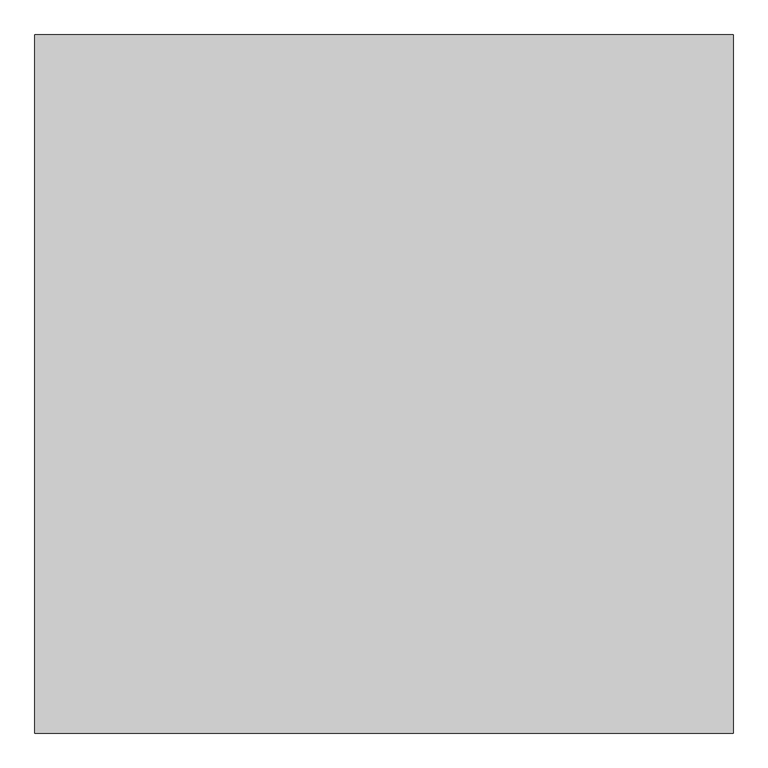
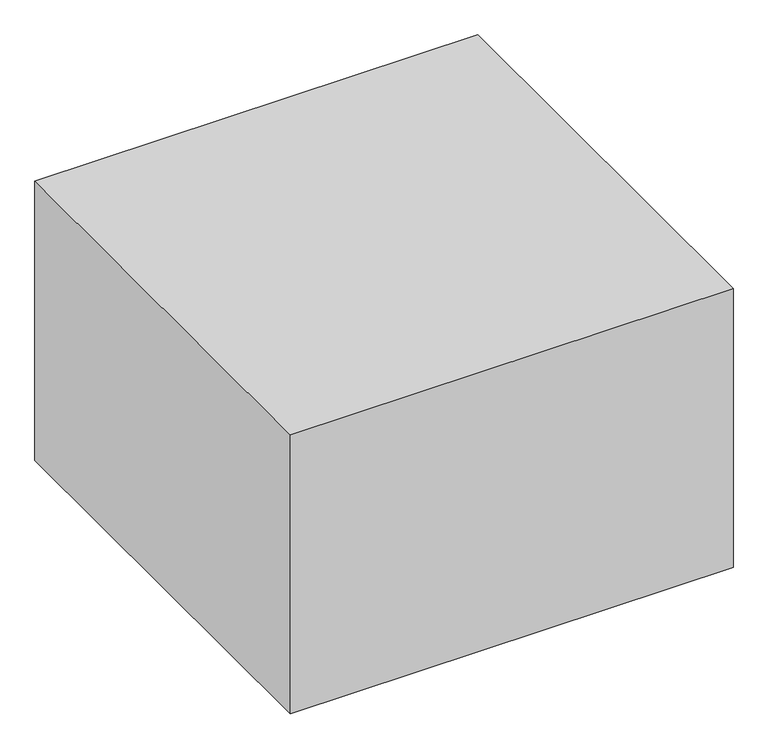
"""IFC4 building model written with IfcOpenShell, lengths in millimetres: proxy geometry, Space Planning Box_hec : Space Planning Box_hec."""

import ifcopenshell
import ifcopenshell.guid

model = None  # the IFC model being written
_history = None  # IfcOwnerHistory: only IFC2X3 demands one
_inside = {}  # id of a spatial element -> (the spatial element, [elements in it])
_under = {}  # id of a project, library or spatial element -> (it, [spatial elements below it])
_declared = {}  # id of a project -> (the project, [libraries it declares])
_typed = {}  # id of a type object -> (the type object, [elements of that type])
_made_of = {}  # id of a material, layer set ... -> (it, [elements and type objects made of it])


def new_model(schema):
    """Start an empty IFC model of exactly this schema.

    Asked for "IFC4X3", IfcOpenShell would pick the latest addendum, in which some entities
    have other attributes; the version numbers below select the first issue.
    IFC2X3 requires an IfcOwnerHistory on every rooted entity: one is made here for all.
    """
    global model, _history
    if schema == "IFC4X3":
        model = ifcopenshell.file(schema_version=(4, 3, 0, 0))
    else:
        model = ifcopenshell.file(schema=schema)
    _inside.clear()
    _under.clear()
    _declared.clear()
    _typed.clear()
    _made_of.clear()
    _history = None
    if model.schema == "IFC2X3":
        org = make("IfcOrganization", Name="unknown")
        user = make(
            "IfcPersonAndOrganization",
            ThePerson=make("IfcPerson", FamilyName="unknown"),
            TheOrganization=org,
        )
        app = make(
            "IfcApplication",
            ApplicationDeveloper=org,
            Version="unknown",
            ApplicationFullName="unknown",
            ApplicationIdentifier="unknown",
        )
        _history = make(
            "IfcOwnerHistory",
            OwningUser=user,
            OwningApplication=app,
            ChangeAction="ADDED",
            CreationDate=0,
        )
    return model


def make(cls, **values):
    """One entity of the class cls with the attributes given. An attribute that is None is left unset."""
    return model.create_entity(
        cls, **{name: value for name, value in values.items() if value is not None}
    )


def rooted(cls, **values):
    """An entity with a GlobalId (a new one), such as an element, a storey or a relation."""
    return make(cls, GlobalId=ifcopenshell.guid.new(), OwnerHistory=_history, **values)


def si_unit(unit_type, name, prefix=None):
    """IfcSIUnit, for example si_unit("LENGTHUNIT", "METRE", prefix="MILLI")."""
    return make("IfcSIUnit", UnitType=unit_type, Prefix=prefix, Name=name)


def assignment(units):
    """IfcUnitAssignment: the units of a project."""
    return None if units is None else make("IfcUnitAssignment", Units=units)


def point(xyz):
    """IfcCartesianPoint."""
    return None if xyz is None else make("IfcCartesianPoint", Coordinates=xyz)


def direction(xyz):
    """IfcDirection."""
    return None if xyz is None else make("IfcDirection", DirectionRatios=xyz)


def frame(location, z_axis=None, x_axis=None):
    """IfcAxis2Placement3D, a coordinate frame: its origin and axes. An axis left out is left unset."""
    return make(
        "IfcAxis2Placement3D",
        Location=point(location),
        Axis=direction(z_axis),
        RefDirection=direction(x_axis),
    )


def origin():
    """The frame at (0, 0, 0) with its axes left unset."""
    return frame((0.0, 0.0, 0.0))


def origin_with_axes():
    """The frame at (0, 0, 0) with the z axis (0, 0, 1) and the x axis (1, 0, 0) written out."""
    return frame((0.0, 0.0, 0.0), z_axis=(0.0, 0.0, 1.0), x_axis=(1.0, 0.0, 0.0))


def place(relative_to, where):
    """IfcLocalPlacement: puts the frame where relative to a parent placement (None: the world)."""
    return make(
        "IfcLocalPlacement", PlacementRelTo=relative_to, RelativePlacement=where
    )


def context(
    kind, dimensions, precision=None, world=None, true_north=None, identifier=None
):
    """IfcGeometricRepresentationContext, for example the 3D "Model" context."""
    return make(
        "IfcGeometricRepresentationContext",
        ContextIdentifier=identifier,
        ContextType=kind,
        CoordinateSpaceDimension=dimensions,
        Precision=precision,
        WorldCoordinateSystem=world,
        TrueNorth=true_north,
    )


def project(units=None, contexts=None):
    """IfcProject with its units and contexts."""
    return rooted(
        "IfcProject",
        Name="project",
        RepresentationContexts=contexts,
        UnitsInContext=assignment(units),
    )


def spatial(cls, under=None, at=None, **own):
    """A site, building, storey or space (cls), placed at a placement, below another one or the project."""
    s = rooted(cls, ObjectPlacement=at, **own)
    if under is not None:
        _under.setdefault(under.id(), (under, []))[1].append(s)
    return s


def polyline(points):
    """IfcPolyline through the points."""
    return make("IfcPolyline", Points=[point(p) for p in points])


def outline(outer, holes=None, kind="AREA"):
    """IfcArbitraryClosedProfileDef: a profile drawn as a closed curve; with holes, ...WithVoids."""
    if holes is None:
        return make("IfcArbitraryClosedProfileDef", ProfileType=kind, OuterCurve=outer)
    return make(
        "IfcArbitraryProfileDefWithVoids",
        ProfileType=kind,
        OuterCurve=outer,
        InnerCurves=holes,
    )


def extrude(swept, where, along, depth):
    """IfcExtrudedAreaSolid: the profile swept, set in the frame where, extruded along a direction by depth."""
    return make(
        "IfcExtrudedAreaSolid",
        SweptArea=swept,
        Position=where,
        ExtrudedDirection=direction(along),
        Depth=depth,
    )


def shape(context_of_items, identifier, shape_type, items):
    """IfcShapeRepresentation: the items that make up one representation, for example the "Body"."""
    return make(
        "IfcShapeRepresentation",
        ContextOfItems=context_of_items,
        RepresentationIdentifier=identifier,
        RepresentationType=shape_type,
        Items=items,
    )


def source(mapping_origin, context_of_items, identifier, shape_type, items):
    """IfcRepresentationMap: a shape defined once, which mapped items show again and again."""
    return make(
        "IfcRepresentationMap",
        MappingOrigin=mapping_origin,
        MappedRepresentation=shape(context_of_items, identifier, shape_type, items),
    )


def transform(
    local_origin,
    x_axis=None,
    y_axis=None,
    z_axis=None,
    scale=None,
    scale2=None,
    scale3=None,
    uniform=True,
):
    """IfcCartesianTransformationOperator3D, or its non-uniform kind. x_axis, y_axis, z_axis: its Axis1, 2, 3."""
    if uniform:
        return make(
            "IfcCartesianTransformationOperator3D",
            Axis1=direction(x_axis),
            Axis2=direction(y_axis),
            LocalOrigin=point(local_origin),
            Scale=scale,
            Axis3=direction(z_axis),
        )
    return make(
        "IfcCartesianTransformationOperator3DnonUniform",
        Axis1=direction(x_axis),
        Axis2=direction(y_axis),
        LocalOrigin=point(local_origin),
        Scale=scale,
        Axis3=direction(z_axis),
        Scale2=scale2,
        Scale3=scale3,
    )


def mapped(mapping_source, mapping_target):
    """IfcMappedItem: shows the shape of a source again, moved by a transform."""
    return make(
        "IfcMappedItem", MappingSource=mapping_source, MappingTarget=mapping_target
    )


def made_of(thing, what):
    """Note that an element or type object is made of a material, layer set ...; save() writes the relation."""
    if what is not None:
        _made_of.setdefault(what.id(), (what, []))[1].append(thing)
    return thing


def element(
    cls,
    number,
    at=None,
    inside=None,
    cuts=None,
    type_object=None,
    material=None,
    context=None,
    identifier="Body",
    shape_type=None,
    held_by="IfcProductDefinitionShape",
    body=None,
    shapes=None,
    **own,
):
    """One element of the class cls, such as IfcWall. Its Tag is "e" and its number.

    at: its placement. inside: the storey or other place that contains it. cuts: it is an
    opening in that element (IfcRelVoidsElement). A single representation is given by context,
    identifier, shape_type and body (its items); several are given by shapes. held_by: the class
    of the entity that holds the representations. save() writes the other relations.
    """
    e = rooted(cls, Tag="e%d" % number, ObjectPlacement=at, **own)
    if body is not None:
        shapes = [shape(context, identifier, shape_type, body)]
    if shapes is not None:
        e.Representation = make(held_by, Representations=shapes)
    if inside is not None:
        _inside.setdefault(inside.id(), (inside, []))[1].append(e)
    if cuts is not None:
        rooted(
            "IfcRelVoidsElement", RelatingBuildingElement=cuts, RelatedOpeningElement=e
        )
    if type_object is not None:
        _typed.setdefault(type_object.id(), (type_object, []))[1].append(e)
    return made_of(e, material)


def aggregate(whole, parts):
    """IfcRelAggregates: a whole, such as a stair, and the parts it consists of."""
    return rooted("IfcRelAggregates", RelatingObject=whole, RelatedObjects=parts)


def save(model, path):
    """Write the relations noted so far, then the file.

    IfcRelAggregates (storeys below a building ...), IfcRelContainedInSpatialStructure (elements
    in a storey), IfcRelDefinesByType, IfcRelAssociatesMaterial and IfcRelDeclares: one each for
    every whole, place, type object, material and project.
    """
    for whole, parts in _under.values():
        aggregate(whole, parts)
    for where, things in _inside.values():
        rooted(
            "IfcRelContainedInSpatialStructure",
            RelatedElements=things,
            RelatingStructure=where,
        )
    for kind, things in _typed.values():
        rooted("IfcRelDefinesByType", RelatedObjects=things, RelatingType=kind)
    for what, things in _made_of.values():
        rooted("IfcRelAssociatesMaterial", RelatedObjects=things, RelatingMaterial=what)
    for by, libraries in _declared.values():
        rooted("IfcRelDeclares", RelatingContext=by, RelatedDefinitions=libraries)
    model.write(path)


def generic_models_b79df083(model_context):
    return source(origin(), model_context, "Body", "SweptSolid", [
        extrude(outline(polyline([(4500.0, 4500.0), (4500.0, -4500.0), (-4500.0, -4500.0), (-4500.0, 4500.0), (4500.0, 4500.0)])), origin_with_axes(), (0.0, 0.0, 1.0), 6000.0),
    ])


if __name__ == "__main__":
    model = new_model("IFC4")
    model_context = context("Model", 3, world=origin())
    ifc_project = project(units=[si_unit("LENGTHUNIT", "METRE", prefix="MILLI")], contexts=[model_context])
    site = spatial("IfcSite", under=ifc_project)
    building = spatial("IfcBuilding", under=site)
    placement = place(None, origin())
    generic_models_shape = generic_models_b79df083(model_context)
    element("IfcBuildingElementProxy", 1, Name="Space Planning Box_hec : Space Planning Box_hec", ObjectType="Space Planning Box_hec : Space Planning Box_hec", at=placement, inside=building, context=model_context, shape_type="MappedRepresentation", body=[
        mapped(generic_models_shape, transform((0.0, 0.0, 0.0), x_axis=(1.0, 0.0, 0.0), y_axis=(0.0, 1.0, 0.0), z_axis=(0.0, 0.0, 1.0))),
    ])
    save(model, "model.ifc")

# Revit data of these elements
# Project information
#   Building Name = "MAIN GATE SECURITY BUILDING"
#   Project Status = "Project Status"
#   Client Name = "현대엔지니어링"
#   Project Address = "서울시 종로구 율곡로 75(계동)"
#   Project Name = "Therma Visayas Energy Project"
#   Project Number = "-"
# Type "Space Planning Box_hec : Space Planning Box_hec"
#   Type Comments = "..."
#   Room Name [instance default] = "?"
#   Interior Finish [instance default] = ""
#   Exterior Finish [instance default] = ""
#   Department [instance default] = ""
#   Assembly Code = "..."
#   Width [instance default] = 1524 mm
#   Program Area [instance default] = 0.00 m²
#   Length [instance default] = 1524 mm
#   Height [instance default] = 1524 mm
#   Area [instance default] = 2.32258 m²
#   Fill Color [instance default] = Cyan
#   Default Elevation = 0
# Element 1 (IfcBuildingElementProxy, "Space Planning Box_hec : Space Planning Box_hec")
#   Room Name = "Kitch & Lunch Room"
#   Interior Finish = "IF2-1"
#   Exterior Finish = "EF1"
#   Department = "AR"
#   Width = 9000 mm
#   Program Area = 31.50 m²
#   Length = 9000 mm
#   Height = 6000 mm
#   Area = 81.00 m²
#   Fill Color = Lavender
#   Materials on its faces: "Lavender"
# Materials
#   "Cyan": class "Generic", colour RGB 0 255 255, transparency 0.2, Cost = 0
#   "Lavender": class "Generic", colour RGB 186 85 211, transparency 0.2, Cost = 0
